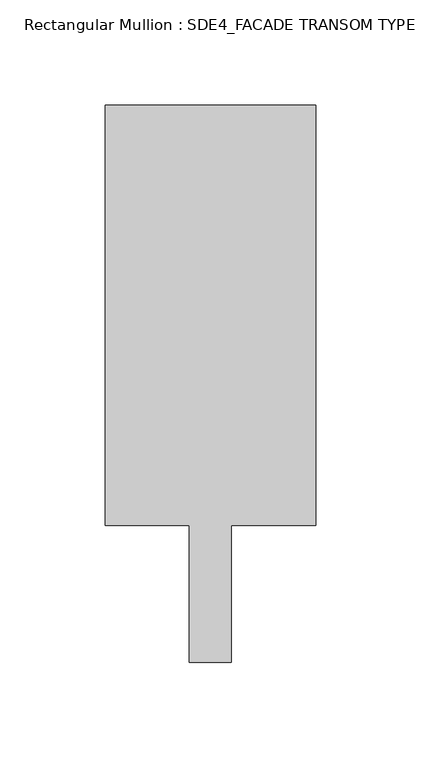
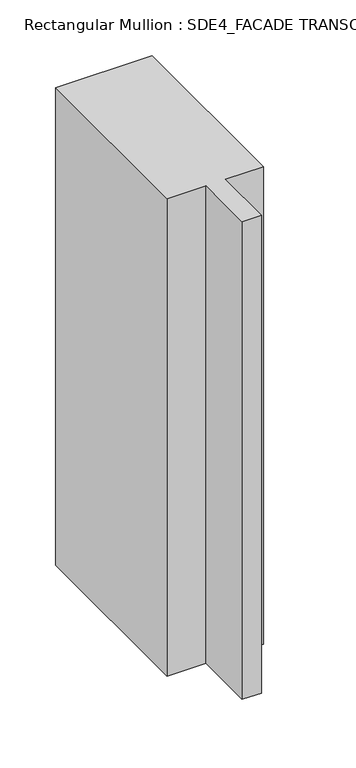
"""IFC4 building model written with IfcOpenShell, lengths in millimetres: member geometry, Rectangular Mullion : SDE4_FACADE TRANSOM TYPE 2."""

from ifc_helpers import new_model, si_unit, frame, origin, place, context, project, spatial, polyline, outline, extrude, source, transform, mapped, element, save


def rectangular_mullion_sde4_facade_transom_type_2_b0441c2b(model_context):
    return source(origin(), model_context, "Body", "SweptSolid", [
        extrude(outline(polyline([(50.0, 132.5), (50.0, -67.5), (10.0, -67.5), (10.0, -132.5), (-10.0, -132.5), (-10.0, -67.5), (-50.0, -67.5), (-50.0, 132.5), (50.0, 132.5)])), frame((0.0, 0.0, -522.5002285), z_axis=(0.0, 0.0, 1.0), x_axis=(1.0, 0.0, 0.0)), (0.0, 0.0, 1.0), 522.5002285),
    ])


if __name__ == "__main__":
    model = new_model("IFC4")
    model_context = context("Model", 3, world=origin())
    ifc_project = project(units=[si_unit("LENGTHUNIT", "METRE", prefix="MILLI")], contexts=[model_context])
    site = spatial("IfcSite", under=ifc_project)
    building = spatial("IfcBuilding", under=site)
    placement = place(None, origin())
    rectangular_mullion_sde4_facade_transom_type_2_shape = rectangular_mullion_sde4_facade_transom_type_2_b0441c2b(model_context)
    element("IfcMember", 1, ObjectType="Rectangular Mullion : SDE4_FACADE TRANSOM TYPE 2", at=placement, inside=building, context=model_context, shape_type="MappedRepresentation", body=[
        mapped(rectangular_mullion_sde4_facade_transom_type_2_shape, transform((0.0, 0.0, 0.0), x_axis=(1.0, 0.0, 0.0), y_axis=(0.0, 1.0, 0.0), z_axis=(0.0, 0.0, 1.0))),
    ])
    save(model, "model.ifc")

# Revit data of these elements
# Type "Rectangular Mullion : SDE4_FACADE TRANSOM TYPE 2"
#   built-in parameter 1007322 = 0.869423 (stored number, unit not read)
#   built-in parameter 1007321 = 0.164042 (stored number, unit not read)
#   built-in parameter 1007320 = 0.164042 (stored number, unit not read)
